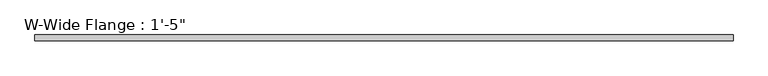
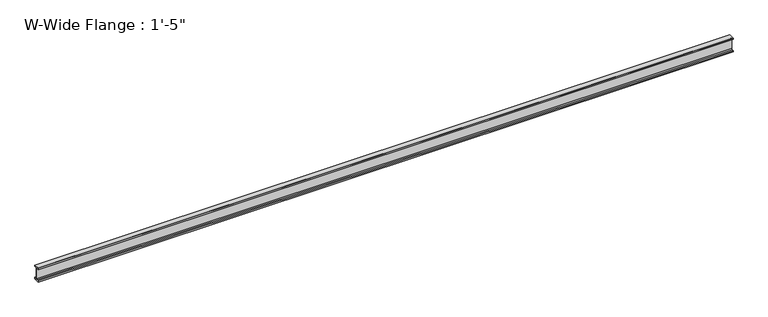
"""IFC4 building model written with IfcOpenShell, lengths in millimetres: beam geometry."""

from ifc_helpers import new_model, si_unit, point, frame, frame_2d, origin, place, context, project, spatial, polyline, circle_curve, trimmed, segment, composite_curve, outline, extrude, source, transform, mapped, element, save


def beam_b6b1cc14(model_context):
    return source(origin(), model_context, "Body", "SweptSolid", [
        extrude(outline(composite_curve([segment(polyline([(76.2, -155.956), (76.2, -190.5), (-76.2, -190.5), (-76.2, -155.956), (-32.131, -155.956)]), True, "CONTINUOUS"), segment(trimmed(circle_curve(frame_2d((-32.131, -133.35)), 22.606), [point((-32.131, -155.956))], [point((-9.525, -133.35))], True, "CARTESIAN"), True, "CONTINUOUS"), segment(polyline([(-9.525, -133.35), (-9.525, 133.35)]), True, "CONTINUOUS"), segment(trimmed(circle_curve(frame_2d((-32.131, 133.35)), 22.606), [point((-9.525, 133.35))], [point((-32.131, 155.956))], True, "CARTESIAN"), True, "CONTINUOUS"), segment(polyline([(-32.131, 155.956), (-76.2, 155.956), (-76.2, 190.5), (76.2, 190.5), (76.2, 155.956), (32.131, 155.956)]), True, "CONTINUOUS"), segment(trimmed(circle_curve(frame_2d((32.131, 133.35)), 22.606), [point((32.131, 155.956))], [point((9.525, 133.35))], True, "CARTESIAN"), True, "CONTINUOUS"), segment(polyline([(9.525, 133.35), (9.525, -133.35)]), True, "CONTINUOUS"), segment(trimmed(circle_curve(frame_2d((32.131, -133.35)), 22.606), [point((9.525, -133.35))], [point((32.131, -155.956))], True, "CARTESIAN"), True, "CONTINUOUS"), segment(polyline([(32.131, -155.956), (76.2, -155.956)]), True, "CONTINUOUS")], self_intersect=False)), frame((-9059.2855518, 0.0, 0.0), z_axis=(1.0, 0.0, 0.0), x_axis=(0.0, 1.0, 0.0)), (0.0, 0.0, 1.0), 18266.7855518),
    ])


if __name__ == "__main__":
    model = new_model("IFC4")
    model_context = context("Model", 3, world=origin())
    ifc_project = project(units=[si_unit("LENGTHUNIT", "METRE", prefix="MILLI")], contexts=[model_context])
    site = spatial("IfcSite", under=ifc_project)
    building = spatial("IfcBuilding", under=site)
    placement = place(None, origin())
    beam_shape = beam_b6b1cc14(model_context)
    element("IfcBeam", 1, ObjectType="W-Wide Flange : 1'-5\"", at=placement, inside=building, context=model_context, shape_type="MappedRepresentation", body=[
        mapped(beam_shape, transform((0.0, 0.0, 0.0), x_axis=(1.0, 0.0, 0.0), y_axis=(0.0, 1.0, 0.0), z_axis=(0.0, 0.0, 1.0))),
    ])
    save(model, "model.ifc")

# Revit data of these elements
# Type "W-Wide Flange : 1'-5\""
#   Assembly Code = "B10"
#   W = 166
#   Length [instance default] = 5' - 0"
#   bf = 0' - 6"
#   d = 1' - 3"
#   k = 0' - 2 1/4"
#   k2 = 0' - 0.89"
#   tf = 0' - 1.36"
#   tw = 0' - 0 3/4"
#   A = 0.338889 SF
#   Structural Material [instance default] = Steel ASTM A992
# Element 1 (IfcBeam, "W-Wide Flange : 1'-5\"")
#   Structural Material = STRUCTURAL STEEL - SEE STRUCT. DWGS
#   Materials on its faces: "STRUCTURAL STEEL - SEE STRUCT. DWGS"
# Materials
#   "Steel ASTM A992": class "Metal", colour RGB 199 199 199, transparency 0, Description = "Structural steel 50ksi", Cost = 0
#   "STRUCTURAL STEEL - SEE STRUCT. DWGS": class "Metal", colour RGB 137 146 153, transparency 0, Description = "Steel, mill finish", Cost = 0
